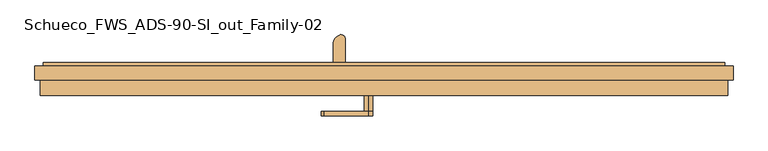
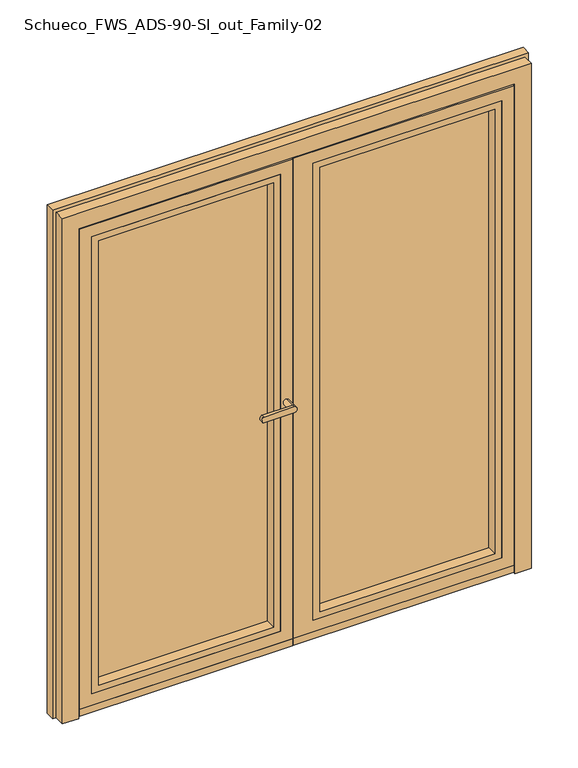
"""IFC4 building model written with IfcOpenShell, lengths in millimetres: door geometry, Schueco_FWS_ADS-90-SI_out_Family-02 : FWS SI insert unit."""

from ifc_helpers import new_model, si_unit, point, frame, frame_2d, origin, place, context, project, spatial, polyline, circle_curve, ellipse_curve, trimmed, segment, composite_curve, outline, extrude, faceted_brep, source, transform, mapped, element, save
from ifc_brep_helpers import plane_surface, cylinder_surface, extruded_surface, advanced_brep


def schueco_fws_ads_90_si_out_family_02_a44193ee(model_context):
    return source(origin(), model_context, "Body", "SolidModel", [
        faceted_brep([(870.0, -72.4997281, 38.0), (870.0, -72.4997281, 2070.0), (870.0, -81.0000038, 2070.0), (870.0, -81.0000038, 38.0), (-12.5, -81.0000038, 38.0), (-12.5, -72.4997281, 38.0), (2.5, -72.4997281, 38.0), (885.0, -72.4997281, 23.0), (885.0, -72.4997281, 2085.0), (2.5, -72.4997281, 2085.0), (2.5, -72.4997281, 2070.0), (2.5, -72.4997281, 23.0), (-12.5, -81.0000038, 2070.0), (65.5, -81.0000038, 86.0), (65.5, -81.0000038, 2022.0), (822.0, -81.0000038, 2022.0), (822.0, -81.0000038, 86.0), (822.0, 0.5000388, 2022.0), (822.0, 0.5000388, 86.0), (65.5, 0.5000388, 86.0), (65.5, 0.5000388, 2022.0), (90.5, 0.5000388, 111.0), (90.5, 0.5000388, 1997.0), (797.0, 0.5000388, 1997.0), (797.0, 0.5000388, 111.0), (797.0, 8.9999962, 1997.0), (797.0, 8.9999962, 111.0), (90.5, 8.9999962, 111.0), (90.5, 8.9999962, 1997.0), (900.0, 8.9999962, 8.0), (17.5, 8.9999962, 8.0), (17.5, 8.9999962, 2100.0), (900.0, 8.9999962, 2100.0), (900.0, 0.5000388, 2100.0), (900.0, 0.5000388, 8.0), (17.5, 0.5000388, 8.0), (17.5, 0.5000388, 2100.0), (17.5, 0.5000388, 2085.0), (885.0, 0.5000388, 2085.0), (885.0, 0.5000388, 23.0), (17.5, 0.5000388, 23.0), (2.5, 0.5000388, 23.0), (2.5, 0.5000388, 2085.0), (-12.5, -72.4997281, 2070.0)], [[[0, 1, 2, 3]], [[3, 4, 5, 6, 0]], [[7, 8, 9, 10, 1, 0, 6, 11]], [[2, 12, 4, 3], [13, 14, 15, 16]], [[16, 15, 17, 18]], [[18, 19, 13, 16]], [[19, 20, 14, 13]], [[18, 17, 20, 19], [21, 22, 23, 24]], [[24, 23, 25, 26]], [[26, 27, 21, 24]], [[27, 28, 22, 21]], [[29, 30, 31, 32], [26, 25, 28, 27]], [[29, 32, 33, 34]], [[34, 35, 30, 29]], [[33, 36, 37, 38, 39, 40, 35, 34]], [[39, 38, 8, 7]], [[7, 11, 41, 40, 39]], [[11, 6, 10, 9, 42, 41]], [[1, 10, 43, 12, 2]], [[20, 17, 15, 14]], [[28, 25, 23, 22]], [[32, 31, 36, 33]], [[9, 8, 38, 37, 42]], [[43, 10, 6, 5]], [[4, 12, 43, 5]], [[37, 36, 31, 30, 35, 40]], [[40, 41, 42, 37]]]),
        extrude(outline(polyline([(86.0, 65.5), (86.0, 822.0), (2022.0, 822.0), (2022.0, 65.5), (86.0, 65.5)]), holes=[polyline([(113.0, 795.0), (113.0, 92.5), (1995.0, 92.5), (1995.0, 795.0), (113.0, 795.0)])]), frame((0.0, -81.0000038, 0.0), z_axis=(0.0, 1.0, 0.0), x_axis=(0.0, 0.0, 1.0)), (0.0, 0.0, 1.0), 43.5000426),
        extrude(outline(polyline([(65.5, -37.4999612), (65.5, 0.5000388), (822.0, 0.5000388), (822.0, -37.4999612), (65.5, -37.4999612)])), frame((0.0, 0.0, 86.0), z_axis=(0.0, 0.0, 1.0), x_axis=(1.0, 0.0, 0.0)), (0.0, 0.0, 1.0), 1936.0),
        extrude(outline(composite_curve([segment(polyline([(-37.1483898, 4.2956275), (-37.1483898, 23.0), (-15.8436573, 23.0), (-15.8436573, 4.2956275)]), True, "CONTINUOUS"), segment(trimmed(circle_curve(frame_2d((-26.4960236, 15.355415)), 15.3555139), [point((-15.8436573, 4.2956275))], [point((-37.1483898, 4.2956275))], False, "CARTESIAN"), True, "CONTINUOUS")], self_intersect=False)), frame((2.5, 0.0, 0.0), z_axis=(1.0, 0.0, 0.0), x_axis=(0.0, 1.0, 0.0)), (0.0, 0.0, 1.0), 882.5),
        extrude(outline(polyline([(870.0, -81.0000038), (-12.5, -81.0000038), (-12.5, -72.4997281), (870.0, -72.4997281), (870.0, -81.0000038)])), frame((0.0, 0.0, 8.0), z_axis=(0.0, 0.0, 1.0), x_axis=(1.0, 0.0, 0.0)), (0.0, 0.0, 1.0), 30.0),
        extrude(outline(composite_curve([segment(polyline([(-139.1673236, 8.9997177), (-139.1673236, 59.1618682)]), True, "CONTINUOUS"), segment(trimmed(circle_curve(frame_2d((-111.9889059, 59.1618682)), 27.1784177), [point((-139.1673236, 59.1618682))], [point((-121.5260015, 84.6120194))], False, "CARTESIAN"), True, "CONTINUOUS"), segment(trimmed(circle_curve(frame_2d((-117.4485005, 73.7310321)), 11.6198924), [point((-121.5260015, 84.6120194))], [point((-105.8286081, 73.7310321))], False, "CARTESIAN"), True, "CONTINUOUS"), segment(polyline([(-105.8286081, 73.7310321), (-105.8286081, 8.9997177), (-139.1673236, 8.9997177)]), True, "CONTINUOUS")], self_intersect=False)), frame((0.0, 0.0, 2043.9340013), z_axis=(0.0, 0.0, 1.0), x_axis=(1.0, 0.0, 0.0)), (0.0, 0.0, 1.0), 4.0),
        extrude(outline(polyline([(-139.1673236, 12.9997177), (-105.8286081, 12.9997177), (-105.8286081, 8.9997177), (-139.1673236, 8.9997177), (-139.1673236, 12.9997177)])), frame((0.0, 0.0, 2013.9340013), z_axis=(0.0, 0.0, 1.0), x_axis=(1.0, 0.0, 0.0)), (0.0, 0.0, 1.0), 30.0),
        extrude(outline(polyline([(-139.1673236, 12.9997177), (-105.8286081, 12.9997177), (-105.8286081, 8.9997177), (-139.1673236, 8.9997177), (-139.1673236, 12.9997177)])), frame((0.0, 0.0, 56.9340013), z_axis=(0.0, 0.0, 1.0), x_axis=(1.0, 0.0, 0.0)), (0.0, 0.0, 1.0), 30.0),
        extrude(outline(composite_curve([segment(polyline([(-139.1673236, 8.9997177), (-139.1673236, 59.1618682)]), True, "CONTINUOUS"), segment(trimmed(circle_curve(frame_2d((-111.9889059, 59.1618682)), 27.1784177), [point((-139.1673236, 59.1618682))], [point((-121.5260015, 84.6120194))], False, "CARTESIAN"), True, "CONTINUOUS"), segment(trimmed(circle_curve(frame_2d((-117.4485005, 73.7310321)), 11.6198924), [point((-121.5260015, 84.6120194))], [point((-105.8286081, 73.7310321))], False, "CARTESIAN"), True, "CONTINUOUS"), segment(polyline([(-105.8286081, 73.7310321), (-105.8286081, 8.9997177), (-139.1673236, 8.9997177)]), True, "CONTINUOUS")], self_intersect=False)), frame((0.0, 0.0, 52.9340013), z_axis=(0.0, 0.0, 1.0), x_axis=(1.0, 0.0, 0.0)), (0.0, 0.0, 1.0), 4.0),
        advanced_brep(
        [(-109.782924, 57.5977179, 2043.9340013), (-135.217076, 72.2821425, 2043.9340013), (-109.782924, 57.5977179, 56.9340013), (-135.217076, 72.2821425, 56.9340013)],
        [
            (0, 1, ellipse_curve(frame((-122.5, 64.9399302, 2043.9340013), z_axis=(0.0, 0.0, 1.0000000000000002), x_axis=(0.5000002582658958, 0.866025254674503, 0.0)), 21.5840887, 14.6844171)),
            (1, 0, ellipse_curve(frame((-122.5, 64.9399302, 2043.9340013), z_axis=(0.0, 0.0, 1.0000000000000002), x_axis=(0.5000002582658958, 0.866025254674503, 0.0)), 21.5840887, 14.6844171)),
            (2, 3, ellipse_curve(frame((-122.5, 64.9399302, 56.9340013), z_axis=(0.0, 0.0, -1.0000000000000002), x_axis=(-0.866025254674503, 0.5000002582658958, 0.0)), 14.6844171, 21.5840887)),
            (3, 2, ellipse_curve(frame((-122.5, 64.9399302, 56.9340013), z_axis=(0.0, 0.0, -1.0000000000000002), x_axis=(-0.866025254674503, 0.5000002582658958, 0.0)), 14.6844171, 21.5840887)),
            (0, 2),
            (3, 1),
        ],
        [
            plane_surface(frame((-135.217076, 72.2821425, 2043.9340013), z_axis=(0.0, 0.0, 1.0000000000000002), x_axis=(0.5000002582658958, 0.866025254674503, 0.0))),
            plane_surface(frame((-135.217076, 72.2821425, 56.9340013), z_axis=(0.0, 0.0, -1.0000000000000002), x_axis=(-0.5000002582658958, -0.866025254674503, 0.0))),
            extruded_surface(trimmed(ellipse_curve(frame((-122.5, 64.9399302, 56.9340013), z_axis=(0.0, 0.0, -1.0000000000000002), x_axis=(-0.866025254674503, 0.5000002582658958, 0.0)), 14.6844171, 21.5840887), [point((-135.217076, 72.2821425, 56.9340013))], [point((-109.782924, 57.5977179, 56.9340013))], True, "CARTESIAN"), (0.0, 0.0, -1987.0), 1987.0),
            extruded_surface(trimmed(ellipse_curve(frame((-122.5, 64.9399302, 56.9340013), z_axis=(0.0, 0.0, -1.0000000000000002), x_axis=(-0.866025254674503, 0.5000002582658958, 0.0)), 14.6844171, 21.5840887), [point((-109.782924, 57.5977179, 56.9340013))], [point((-135.217076, 72.2821425, 56.9340013))], True, "CARTESIAN"), (0.0, 0.0, -1987.0), 1987.0),
        ],
        [
            (0, [[1, 2]]),
            (1, [[3, 4]]),
            (2, [[5, -4, 6, -1]]),
            (3, [[-6, -3, -5, -2]]),
        ],
    ),
        advanced_brep(
        [(-42.5, -137.0002518, 1038.0113692), (-42.5, -137.0002518, 1061.9886308), (-164.1617926, -137.0002518, 1061.9886308), (-164.1617926, -137.0002518, 1038.0113692), (-42.5, -124.5001648, 1061.9886308), (-42.5, -124.5001648, 1038.0113692), (-164.1617926, -124.5001648, 1038.0113692), (-164.1617926, -124.5001648, 1061.9886308), (-42.5, -81.0002823, 1038.0113692), (-42.5, -81.0002823, 1061.9886308)],
        [
            (0, 1, circle_curve(frame((-42.5, -137.0002518, 1050.0), z_axis=(0.0, -1.0, 0.0), x_axis=(0.0, 0.0, 1.0)), 11.9886308)),
            (1, 2),
            (2, 3, ellipse_curve(frame((-164.1617926, -137.0002518, 1050.0), z_axis=(0.0, -1.0, 0.0), x_axis=(0.0, 0.0, -1.0)), 11.9886308, 7.9050795)),
            (3, 0),
            (4, 5, circle_curve(frame((-42.5, -124.5001648, 1050.0), z_axis=(0.0, -1.0, 0.0), x_axis=(0.0, 0.0, 1.0)), 11.9886308)),
            (5, 6),
            (6, 7, ellipse_curve(frame((-164.1617926, -124.5001648, 1050.0), z_axis=(0.0, 1.0, 0.0), x_axis=(0.0, 0.0, -1.0)), 11.9886308, 7.9050795)),
            (7, 4),
            (3, 6),
            (5, 0),
            (2, 7),
            (1, 4),
            (5, 4, circle_curve(frame((-42.5, -124.5001648, 1050.0), z_axis=(0.0, -1.0, 0.0), x_axis=(0.0, 0.0, 1.0)), 11.9886308)),
            (8, 9, circle_curve(frame((-42.5, -81.0002823, 1050.0), z_axis=(0.0, 1.0, 0.0), x_axis=(0.0, 0.0, 1.0)), 11.9886308)),
            (9, 8, circle_curve(frame((-42.5, -81.0002823, 1050.0), z_axis=(0.0, 1.0, 0.0), x_axis=(0.0, 0.0, 1.0)), 11.9886308)),
            (8, 5),
            (4, 9),
        ],
        [
            plane_surface(frame((-164.1617926, -137.0002518, 1038.0113692), z_axis=(0.0, -1.0, 0.0), x_axis=(-1.0, 0.0, 0.0))),
            plane_surface(frame((-164.1617926, -124.5001648, 1038.0113692), z_axis=(0.0, 1.0, 0.0), x_axis=(1.0, 0.0, 0.0))),
            plane_surface(frame((-42.5, -137.0002518, 1038.0113692), z_axis=(0.0, 0.0, -1.0), x_axis=(0.0, 1.0, 0.0))),
            extruded_surface(trimmed(ellipse_curve(frame((-164.1617926, -124.5001648, 1050.0), z_axis=(0.0, 1.0, 0.0), x_axis=(0.0, 0.0, -1.0)), 11.9886308, 7.9050795), [point((-164.1617926, -124.5001648, 1038.0113692))], [point((-164.1617926, -124.5001648, 1061.9886308))], True, "CARTESIAN"), (0.0, 12.500086999999994, 0.0), 12.500086999999994),
            plane_surface(frame((-164.1617926, -137.0002518, 1061.9886308), z_axis=(0.0, 0.0, 1.0), x_axis=(0.0, 1.0, 0.0))),
            cylinder_surface(frame((-42.5, -124.5001648, 1050.0), z_axis=(0.0, -1.0, 0.0), x_axis=(0.0, 0.0, 1.0)), 11.9886308),
            plane_surface(frame((-42.5, -81.0002823, 1061.9886308), z_axis=(0.0, 1.0, 0.0), x_axis=(-1.0, 0.0, 0.0))),
            cylinder_surface(frame((-42.5, -81.0002823, 1050.0), z_axis=(0.0, -1.0, 0.0), x_axis=(0.0, 0.0, 1.0)), 11.9886308),
        ],
        [
            (0, [[1, 2, 3, 4]]),
            (1, [[5, 6, 7, 8]]),
            (2, [[9, -6, 10, -4]]),
            (3, [[11, -7, -9, -3]]),
            (4, [[12, -8, -11, -2]]),
            (5, [[-10, 13, -12, -1]]),
            (6, [[14, 15]]),
            (7, [[16, -5, 17, -14]]),
            (7, [[-17, -13, -16, -15]]),
        ],
    ),
        faceted_brep([(-870.0, -72.5000065, 38.0), (-870.0, -81.0002823, 38.0), (-870.0, -81.0002823, 2070.0), (-870.0, -72.5000065, 2070.0), (-19.5, -72.5000065, 38.0), (-17.5, -72.5000065, 38.0), (-17.5, -81.0002823, 38.0), (-19.5, -81.0002823, 38.0), (-885.0, -72.5000065, 23.0), (-2.5, -72.5000065, 23.0), (-2.5, -72.5000065, 2085.0), (-885.0, -72.5000065, 2085.0), (-17.5, -72.5000065, 2070.0), (-19.5, -72.5000065, 2070.0), (-17.5, -81.0002823, 2070.0), (-19.5, -81.0002823, 2070.0), (-65.5, -81.0002823, 86.0), (-822.0, -81.0002823, 86.0), (-822.0, -81.0002823, 2022.0), (-65.5, -81.0002823, 2022.0), (-822.0, 0.4997603, 86.0), (-822.0, 0.4997603, 2022.0), (-65.5, 0.4997603, 86.0), (-65.5, 0.4997603, 2022.0), (-90.5, 0.4997603, 111.0), (-797.0, 0.4997603, 111.0), (-797.0, 0.4997603, 1997.0), (-90.5, 0.4997603, 1997.0), (-797.0, 8.9997177, 111.0), (-797.0, 8.9997177, 1997.0), (-90.5, 8.9997177, 111.0), (-90.5, 8.9997177, 1997.0), (12.5, 8.9997177, 8.0), (-900.0, 8.9997177, 8.0), (-900.0, 8.9997177, 2100.0), (12.5, 8.9997177, 2100.0), (-900.0, 0.4997603, 8.0), (-900.0, 0.4997603, 2100.0), (12.5, 0.4997603, 8.0), (12.5, 0.4997603, 2100.0), (-2.5, 0.4997603, 23.0), (-885.0, 0.4997603, 23.0), (-885.0, 0.4997603, 2085.0), (-2.5, 0.4997603, 2085.0)], [[[0, 1, 2, 3]], [[1, 0, 4, 5, 6, 7]], [[8, 9, 10, 11], [12, 5, 4, 0, 3, 13]], [[6, 5, 12, 14]], [[6, 14, 15, 2, 1, 7], [16, 17, 18, 19]], [[17, 20, 21, 18]], [[20, 17, 16, 22]], [[22, 16, 19, 23]], [[20, 22, 23, 21], [24, 25, 26, 27]], [[25, 28, 29, 26]], [[28, 25, 24, 30]], [[30, 24, 27, 31]], [[32, 33, 34, 35], [28, 30, 31, 29]], [[33, 36, 37, 34]], [[36, 33, 32, 38]], [[38, 32, 35, 39]], [[36, 38, 39, 37], [40, 41, 42, 43]], [[41, 8, 11, 42]], [[8, 41, 40, 9]], [[9, 40, 43, 10]], [[14, 12, 13, 3, 2, 15]], [[23, 19, 18, 21]], [[31, 27, 26, 29]], [[39, 35, 34, 37]], [[10, 43, 42, 11]]]),
        extrude(outline(polyline([(86.0, -65.5), (2022.0, -65.5), (2022.0, -822.0), (86.0, -822.0), (86.0, -65.5)]), holes=[polyline([(113.0, -795.0), (1995.0, -795.0), (1995.0, -92.5), (113.0, -92.5), (113.0, -795.0)])]), frame((0.0, -81.0002823, 0.0), z_axis=(0.0, 1.0, 0.0), x_axis=(0.0, 0.0, 1.0)), (0.0, 0.0, 1.0), 43.5000426),
        extrude(outline(polyline([(-65.5, -37.5002397), (-822.0, -37.5002397), (-822.0, 0.4997603), (-65.5, 0.4997603), (-65.5, -37.5002397)])), frame((0.0, 0.0, 86.0), z_axis=(0.0, 0.0, 1.0), x_axis=(1.0, 0.0, 0.0)), (0.0, 0.0, 1.0), 1936.0),
        extrude(outline(composite_curve([segment(polyline([(-37.1486683, 4.2956275), (-37.1486683, 23.0), (-15.8439358, 23.0), (-15.8439358, 4.2956275)]), True, "CONTINUOUS"), segment(trimmed(circle_curve(frame_2d((-26.496302, 15.355415)), 15.3555139), [point((-15.8439358, 4.2956275))], [point((-37.1486683, 4.2956275))], False, "CARTESIAN"), True, "CONTINUOUS")], self_intersect=False)), frame((-885.0, 0.0, 0.0), z_axis=(1.0, 0.0, 0.0), x_axis=(0.0, 1.0, 0.0)), (0.0, 0.0, 1.0), 882.5),
        extrude(outline(polyline([(-870.0, -81.0002823), (-870.0, -72.5000065), (-17.5, -72.5000065), (-17.5, -81.0002823), (-870.0, -81.0002823)])), frame((0.0, 0.0, 8.0), z_axis=(0.0, 0.0, 1.0), x_axis=(1.0, 0.0, 0.0)), (0.0, 0.0, 1.0), 30.0),
        faceted_brep([(930.999943, 8.9997177, 2130.999943), (930.999943, 0.0, 2130.999943), (930.999943, 0.0, 0.0), (930.999943, 8.9997177, 0.0), (-954.0, 0.0, 0.0), (-954.0, 0.0, 2154.0), (954.0, 0.0, 2154.0), (954.0, 0.0, 0.0), (-930.999943, 0.0, 2130.999943), (-930.999943, 0.0, 0.0), (954.0, -38.0, 0.0), (940.0, -38.0, 0.0), (940.0, -81.0002823, 0.0), (875.0652914, -81.0002823, 0.0), (875.0652914, -72.5000065, 0.0), (893.4999114, -72.5000065, 0.0), (893.4999114, 0.4997603, 0.0), (904.9999827, 0.4997603, 0.0), (904.9999827, 8.9997177, 0.0), (-904.9999827, 8.9997177, 0.0), (-930.999943, 8.9997177, 0.0), (-930.999943, 8.9997177, 2130.999943), (904.9999827, 8.9997177, 2104.9999827), (-904.9999827, 8.9997177, 2104.9999827), (875.0652914, -81.0002823, 2075.0652914), (875.0652914, -72.5000065, 2075.0652914), (-875.0652914, -72.5000065, 0.0), (-893.4999114, -72.5000065, 0.0), (-893.4999114, -72.5000065, 2093.4999114), (893.4999114, -72.5000065, 2093.4999114), (-875.0652914, -72.5000065, 2075.0652914), (-940.0, -81.0002823, 0.0), (-875.0652914, -81.0002823, 0.0), (-875.0652914, -81.0002823, 2075.0652914), (940.0, -81.0002823, 2140.0), (-940.0, -81.0002823, 2140.0), (940.0, -38.0, 2140.0), (-954.0, -38.0, 0.0), (-940.0, -38.0, 0.0), (-940.0, -38.0, 2140.0), (954.0, -38.0, 2154.0), (-954.0, -38.0, 2154.0), (-904.9999827, 0.4997603, 0.0), (-893.4999114, 0.4997603, 0.0), (904.9999827, 0.4997603, 2104.9999827), (-904.9999827, 0.4997603, 2104.9999827), (893.4999114, 0.4997603, 2093.4999114), (-893.4999114, 0.4997603, 2093.4999114)], [[[0, 1, 2, 3]], [[4, 5, 6, 7, 2, 1, 8, 9]], [[3, 2, 7, 10, 11, 12, 13, 14, 15, 16, 17, 18]], [[19, 20, 21, 0, 3, 18, 22, 23]], [[24, 25, 14, 13]], [[26, 27, 28, 29, 15, 14, 25, 30]], [[31, 32, 33, 24, 13, 12, 34, 35]], [[34, 12, 11, 36]], [[37, 38, 39, 36, 11, 10, 40, 41]], [[4, 9, 20, 19, 42, 43, 27, 26, 32, 31, 38, 37]], [[20, 9, 8, 21]], [[18, 17, 44, 22]], [[42, 19, 23, 45]], [[32, 26, 30, 33]], [[31, 35, 39, 38]], [[4, 37, 41, 5]], [[6, 40, 10, 7]], [[43, 42, 45, 44, 17, 16, 46, 47]], [[16, 15, 29, 46]], [[27, 43, 47, 28]], [[21, 8, 1, 0]], [[33, 30, 25, 24]], [[35, 34, 36, 39]], [[23, 22, 44, 45]], [[5, 41, 40, 6]], [[47, 46, 29, 28]]]),
    ])


if __name__ == "__main__":
    model = new_model("IFC4")
    model_context = context("Model", 3, world=origin())
    ifc_project = project(units=[si_unit("LENGTHUNIT", "METRE", prefix="MILLI")], contexts=[model_context])
    site = spatial("IfcSite", under=ifc_project)
    building = spatial("IfcBuilding", under=site)
    placement = place(None, origin())
    schueco_fws_ads_90_si_out_family_02_shape = schueco_fws_ads_90_si_out_family_02_a44193ee(model_context)
    element("IfcDoor", 1, ObjectType="Schueco_FWS_ADS-90-SI_out_Family-02 : FWS SI insert unit", at=placement, inside=building, context=model_context, shape_type="MappedRepresentation", body=[
        mapped(schueco_fws_ads_90_si_out_family_02_shape, transform((0.0, 0.0, 0.0), x_axis=(1.0, 0.0, 0.0), y_axis=(0.0, 1.0, 0.0), z_axis=(0.0, 0.0, 1.0))),
    ])
    save(model, "model.ifc")

# Revit data of these elements
# Type "Schueco_FWS_ADS-90-SI_out_Family-02 : FWS SI insert unit"
#   Type Mark = "58"
#   __NOTE__ = "Data describes the optimum values of the entire system. The properites of a selected design option have to be determined on an individual basis!"
#   Wind load resistance = "Class C3"
#   Watertightness = "Class 7A"
#   Thermal insulation = "Uf = 1.2 W/(m²K)"
#   Sound insulation = "..."
#   Schueco thermal insulation standard = "Highly thermally insulated"
#   Opening type = "Outward-opening, Flush-fitted"
#   Model = "Schueco ADS 90.SI"
#   Mechanical loading = "Class 3"
#   Maximum leaf width in mm = "1400"
#   Maximum leaf weight in kg = "160"
#   Maximum leaf height in mm = "2500"
#   Material = "Aluminium"
#   Long term functionality = "..."
#   Construction Type = "Door, double-leaf, outward-opening"
#   Manufacturer = "Schueco International KG"
#   Glazing data = "Triple glazing 38mm"
#   Façade insert unit = "yes"
#   Family creation date = "08.2017"
#   Description = "Schueco Aluminium Door System (ADS)"
#   Burglar resistance = "Class RC 3"
#   Areas of use = "Public buildings, Side entrance"
#   Analytic Construction = "<None>"
#   Air permeability = "Class 4"
#   Width [instance default] = 1268.272 mm
#   Leaf opening angle [instance default] = 0.00°
#   IOf_T = 38 mm
#   Height [instance default] = 2054.517 mm
#   Glazing area [instance default] = 1.36411 m²
#   F2_W [instance default] = 634.136 mm
#   F1_W [instance default] = 634.136 mm
#   Distance from bottom to handles [instance default] = 1050 mm
#   Clear opening width [instance default] = 1110.272 mm
#   Active leaf width = 800 mm
#   Standard threshold = no
#   Low level threshold = yes
#   Handles = yes
#   All fields of identical width = yes
#   Glass = none
#   Frame = Alu
#   Fittings = none
# Element 1 (IfcDoor, "Schueco_FWS_ADS-90-SI_out_Family-02 : FWS SI insert unit")
#   Width = 1908 mm
#   Height = 2154 mm
#   Glazing area = 2.64421 m²
#   F2_W = 954 mm
#   F1_W = 954 mm
#   Clear opening width = 1750 mm
#   Materials on its faces: "Alu", "Glass"
# Materials
#   "Alu": class "Glas", colour RGB 140 140 140, transparency 0
#   "Glass": class "Glass", colour RGB 128 128 255, transparency 0.75, Description = "Soda Lime Glass", Cost = 0
